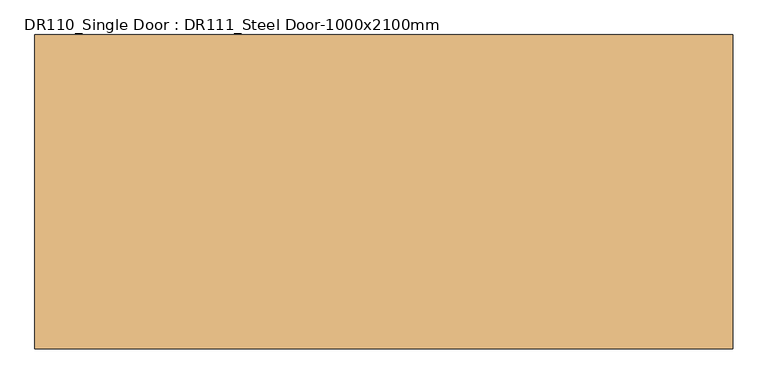
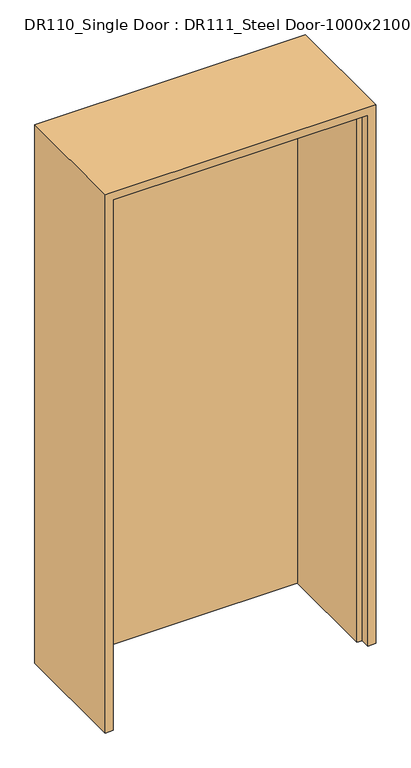
"""IFC4 building model written with IfcOpenShell, lengths in millimetres: door geometry, DR110_Single Door : DR111_Steel Door-1000x2100mm."""

from ifc_helpers import new_model, si_unit, origin, origin_with_axes, place, context, project, spatial, polyline, outline, extrude, faceted_brep, source, transform, mapped, element, save


def dr110_single_door_dr111_steel_door_1000x2100mm_e52ce95f(model_context):
    return source(origin(), model_context, "Body", "SolidModel", [
        extrude(outline(polyline([(470.0, 225.0), (470.0, 190.0), (-470.0, 190.0), (-470.0, 225.0), (470.0, 225.0)])), origin_with_axes(), (0.0, 0.0, 1.0), 2070.0),
        faceted_brep([(470.0, 225.0, 0.0), (500.0, 225.0, 0.0), (500.0, -225.0, 0.0), (470.0, -225.0, 0.0), (470.0, -190.0, 0.0), (450.0, -190.0, 0.0), (450.0, 190.0, 0.0), (470.0, 190.0, 0.0), (470.0, 225.0, 2070.0), (-470.0, 225.0, 2070.0), (-470.0, 225.0, 0.0), (-500.0, 225.0, 0.0), (-500.0, 225.0, 2100.0), (500.0, 225.0, 2100.0), (500.0, -225.0, 2100.0), (-500.0, -225.0, 2100.0), (-500.0, -225.0, 0.0), (-470.0, -225.0, 0.0), (-470.0, -225.0, 2070.0), (470.0, -225.0, 2070.0), (470.0, -190.0, 2070.0), (-470.0, -190.0, 2070.0), (-470.0, -190.0, 0.0), (-450.0, -190.0, 0.0), (-450.0, -190.0, 2050.0), (450.0, -190.0, 2050.0), (450.0, 190.0, 2050.0), (-450.0, 190.0, 2050.0), (-450.0, 190.0, 0.0), (-470.0, 190.0, 0.0), (-470.0, 190.0, 2070.0), (470.0, 190.0, 2070.0)], [[[0, 1, 2, 3, 4, 5, 6, 7]], [[1, 0, 8, 9, 10, 11, 12, 13]], [[2, 1, 13, 14]], [[3, 2, 14, 15, 16, 17, 18, 19]], [[4, 3, 19, 20]], [[5, 4, 20, 21, 22, 23, 24, 25]], [[6, 5, 25, 26]], [[7, 6, 26, 27, 28, 29, 30, 31]], [[0, 7, 31, 8]], [[9, 30, 29, 10]], [[10, 29, 28, 23, 22, 17, 16, 11]], [[15, 12, 11, 16]], [[21, 18, 17, 22]], [[27, 24, 23, 28]], [[14, 13, 12, 15]], [[20, 19, 18, 21]], [[26, 25, 24, 27]], [[8, 31, 30, 9]]]),
    ])


if __name__ == "__main__":
    model = new_model("IFC4")
    model_context = context("Model", 3, world=origin())
    ifc_project = project(units=[si_unit("LENGTHUNIT", "METRE", prefix="MILLI")], contexts=[model_context])
    site = spatial("IfcSite", under=ifc_project)
    building = spatial("IfcBuilding", under=site)
    placement = place(None, origin())
    dr110_single_door_dr111_steel_door_1000x2100mm_shape = dr110_single_door_dr111_steel_door_1000x2100mm_e52ce95f(model_context)
    element("IfcDoor", 1, ObjectType="DR110_Single Door : DR111_Steel Door-1000x2100mm", at=placement, inside=building, context=model_context, shape_type="MappedRepresentation", body=[
        mapped(dr110_single_door_dr111_steel_door_1000x2100mm_shape, transform((0.0, 0.0, 0.0), x_axis=(1.0, 0.0, 0.0), y_axis=(0.0, 1.0, 0.0), z_axis=(0.0, 0.0, 1.0))),
    ])
    save(model, "model.ifc")

# Revit data of these elements
# Type "DR110_Single Door : DR111_Steel Door-1000x2100mm"
#   Type Mark = "SD"
#   Analytic Construction = "<None>"
#   프레임 투영 외부. = 25 mm
#   프레임 투영 내부. = 25 mm
#   프레임 폭 = 75 mm
#   Height = 2100 mm
#   Width = 1000 mm
#   Define Thermal Properties by = 1
#   문 패널 = SD1 문 패널
#   문 프레임 = A04AQ098-00002_Steel Door_non FP_single
#   Function = (empty or 0)
#   Wall Closure = (empty or 0)
# Element 1 (IfcDoor, "DR110_Single Door : DR111_Steel Door-1000x2100mm")
#   Materials on its faces: "A04AQ098-00002_Steel Door_non FP_single", "SD1 문 패널"
# Materials
#   "SD1 문 패널": class "금속", colour RGB 247 247 247, transparency 0, Description = "STEEL DOOR (1000Wx2100H)"
#   "A04AQ098-00002_Steel Door_non FP_single": class "금속", colour RGB 247 247 247, transparency 0, Description = "Steel Door", W00) Work Master Code = "A04AQ098-00002", W01) Work Master_Lv1 = "Finishing Work", W02) Work Master_Lv2 = "Door & Window Work", W03) Work Master_Spec.1 = "Steel Door w/ Steel Frame", W04) Work Master_Spec.2 = "Fire Protective Rating: N/A, Single Door", W05) Work Master_Spec.3 = "w/ Hardware & Accessories", Cost = 0
